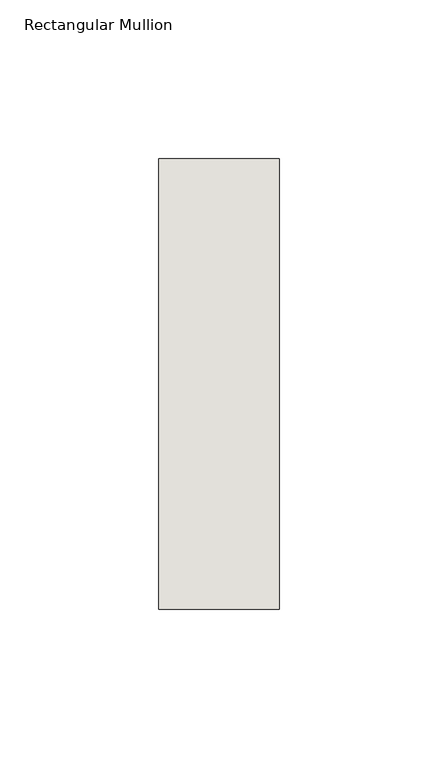
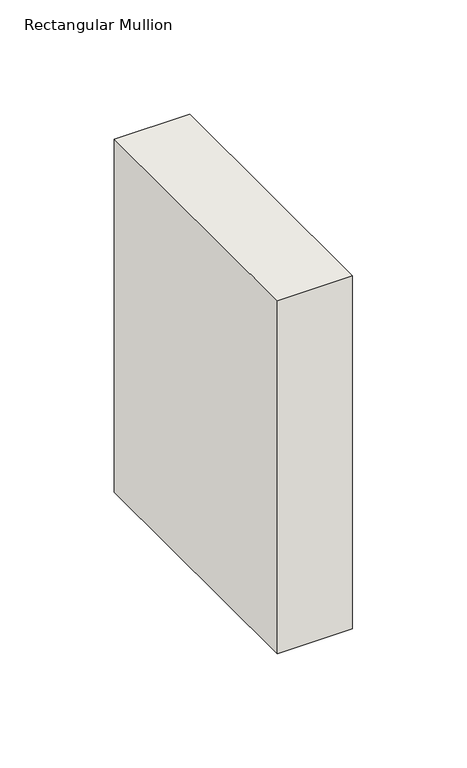
"""IFC4 building model written with IfcOpenShell, lengths in millimetres: wall geometry, Rectangular Mullion : NLRS_21_CWM_hsb-regel 38x142_gen_rsf."""

from ifc_helpers import new_model, si_unit, frame, origin, place, context, project, spatial, polyline, outline, extrude, source, transform, mapped, element, save


def rectangular_mullion_45cc79de(model_context):
    return source(origin(), model_context, "Body", "SweptSolid", [
        extrude(outline(polyline([(-38.0, -71.0), (-38.0, 71.0), (0.0, 71.0), (0.0, -71.0), (-38.0, -71.0)])), frame((0.0, 0.0, -188.0000003), z_axis=(0.0, 0.0, 1.0), x_axis=(1.0, 0.0, 0.0)), (0.0, 0.0, 1.0), 188.0000003),
    ])


if __name__ == "__main__":
    model = new_model("IFC4")
    model_context = context("Model", 3, world=origin())
    ifc_project = project(units=[si_unit("LENGTHUNIT", "METRE", prefix="MILLI")], contexts=[model_context])
    site = spatial("IfcSite", under=ifc_project)
    building = spatial("IfcBuilding", under=site)
    placement = place(None, origin())
    rectangular_mullion_shape = rectangular_mullion_45cc79de(model_context)
    element("IfcWall", 1, ObjectType="Rectangular Mullion : NLRS_21_CWM_hsb-regel 38x142_gen_rsf", at=placement, inside=building, context=model_context, shape_type="MappedRepresentation", body=[
        mapped(rectangular_mullion_shape, transform((0.0, 0.0, 0.0), x_axis=(1.0, 0.0, 0.0), y_axis=(0.0, 1.0, 0.0), z_axis=(0.0, 0.0, 1.0))),
    ])
    save(model, "model.ifc")

# Revit data of these elements
# Type "Rectangular Mullion : NLRS_21_CWM_hsb-regel 38x142_gen_rsf"
#   Type IfcGUID = "07M7mRoiH1CR8m_RSKIwpF"
#   Assembly Code = "21.10"
#   IfcExportAs = "IfcWall"
#   built-in parameter 1007322 = 0.465879 (stored number, unit not read)
#   built-in parameter 1007321 = 0.062336 (stored number, unit not read)
#   built-in parameter 1007320 = 0.062336 (stored number, unit not read)
# Element 1 (IfcWall, "Rectangular Mullion : NLRS_21_CWM_hsb-regel 38x142_gen_rsf")
#   Materials on its faces: "NLRS_i2_hout naaldhout vuren_gen_rsf"
# Materials
#   "NLRS_i2_hout naaldhout vuren_gen_rsf": class "I - Hout", colour RGB 234 199 147, transparency 0, Keynote = "i2", Manufacturer = "Revit Standards Foundation", URL = "www.revitstandards.org", Description = "hout vuren", Cost = 0
